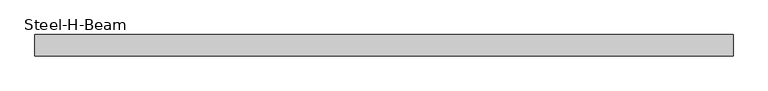
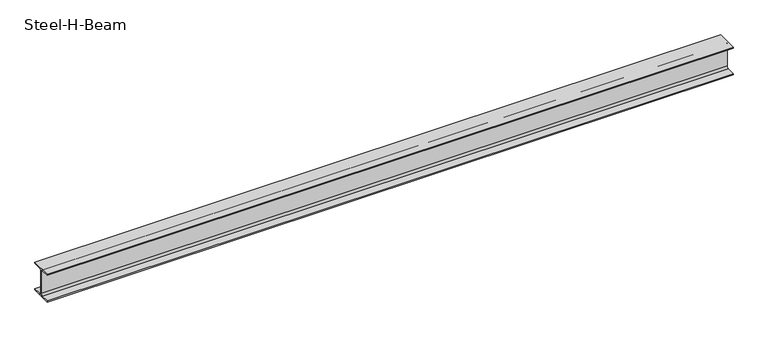
"""IFC4 building model written with IfcOpenShell, lengths in millimetres: beam geometry, Steel-H-Beam : BM121_H-244×175x7x11."""

from ifc_helpers import new_model, si_unit, point, frame, frame_2d, origin, place, context, project, spatial, polyline, circle_curve, trimmed, segment, composite_curve, outline, extrude, source, transform, mapped, element, save


def steel_h_beam_2cee67ca(model_context):
    return source(origin(), model_context, "Body", "SweptSolid", [
        extrude(outline(composite_curve([segment(polyline([(87.5, -111.0), (87.5, -122.0), (-87.5, -122.0), (-87.5, -111.0), (-19.5, -111.0)]), True, "CONTINUOUS"), segment(trimmed(circle_curve(frame_2d((-19.5, -95.0)), 16.0), [point((-19.5, -111.0))], [point((-3.5, -95.0))], True, "CARTESIAN"), True, "CONTINUOUS"), segment(polyline([(-3.5, -95.0), (-3.5, 95.0)]), True, "CONTINUOUS"), segment(trimmed(circle_curve(frame_2d((-19.5, 95.0)), 16.0), [point((-3.5, 95.0))], [point((-19.5, 111.0))], True, "CARTESIAN"), True, "CONTINUOUS"), segment(polyline([(-19.5, 111.0), (-87.5, 111.0), (-87.5, 122.0), (87.5, 122.0), (87.5, 111.0), (19.5, 111.0)]), True, "CONTINUOUS"), segment(trimmed(circle_curve(frame_2d((19.5, 95.0)), 16.0), [point((19.5, 111.0))], [point((3.5, 95.0))], True, "CARTESIAN"), True, "CONTINUOUS"), segment(polyline([(3.5, 95.0), (3.5, -95.0)]), True, "CONTINUOUS"), segment(trimmed(circle_curve(frame_2d((19.5, -95.0)), 16.0), [point((3.5, -95.0))], [point((19.5, -111.0))], True, "CARTESIAN"), True, "CONTINUOUS"), segment(polyline([(19.5, -111.0), (87.5, -111.0)]), True, "CONTINUOUS")], self_intersect=False)), frame((-2886.3486745, 0.0, 0.0), z_axis=(1.0, 0.0, 0.0), x_axis=(0.0, 1.0, 0.0)), (0.0, 0.0, 1.0), 5681.8597388),
    ])


if __name__ == "__main__":
    model = new_model("IFC4")
    model_context = context("Model", 3, world=origin())
    ifc_project = project(units=[si_unit("LENGTHUNIT", "METRE", prefix="MILLI")], contexts=[model_context])
    site = spatial("IfcSite", under=ifc_project)
    building = spatial("IfcBuilding", under=site)
    placement = place(None, origin())
    steel_h_beam_shape = steel_h_beam_2cee67ca(model_context)
    element("IfcBeam", 1, ObjectType="Steel-H-Beam : BM121_H-244×175x7x11", at=placement, inside=building, context=model_context, shape_type="MappedRepresentation", body=[
        mapped(steel_h_beam_shape, transform((0.0, 0.0, 0.0), x_axis=(1.0, 0.0, 0.0), y_axis=(0.0, 1.0, 0.0), z_axis=(0.0, 0.0, 1.0))),
    ])
    save(model, "model.ifc")

# Revit data of these elements
# Type "Steel-H-Beam : BM121_H-244×175x7x11"
#   Surface Area = 1.14653 m²/m
#   Section Area = 56.2375 cm²
#   Mass per Unit Length = 44.1465 kg/m
#   Length [instance default] = 3000 mm
#   B = 175 mm
#   H = 244 mm
#   r = 16 mm
#   tw = 7 mm
#   tf = 11 mm
#   hec_material4 [instance default] = none
#   hec_material3 [instance default] = none
#   hec_material2 [instance default] = none
#   hec_material1 [instance default] = none
#   Structural Material [instance default] = Steel, 45-345
#   Assembly Code = ""
# Element 1 (IfcBeam, "Steel-H-Beam : BM121_H-244×175x7x11")
#   Structural Material = S03AA028-00001_Main Steel Structure Erection Work_Shelter/Building_Medium Steel
#   Materials on its faces: "S03AA028-00001_Main Steel Structure Erection Work_Shelter/Building_Medium Steel"
# Materials
#   "Steel, 45-345": class "Metal", colour RGB 189 187 185, transparency 0, Description = "Steel 345 MPa", Cost = 0
#   "S03AA028-00001_Main Steel Structure Erection Work_Shelter/Building_Medium Steel": class "Metal", colour RGB 120 120 120, transparency 0, Comments = "(90KG/M>Weight≥30KG/M)", Description = "Structural steel 50ksi", W00) Work Master Code = "S03AA028-0001", W01) Work Master_Lv1 = "Main Steel Structure Erection Work", W02) Work Master_Lv2 = "Shelter/Building", W03) Work Master_Spec.1 = "Medium Steel (90KG/M>Weight≥30KG/M)", Cost = 0
